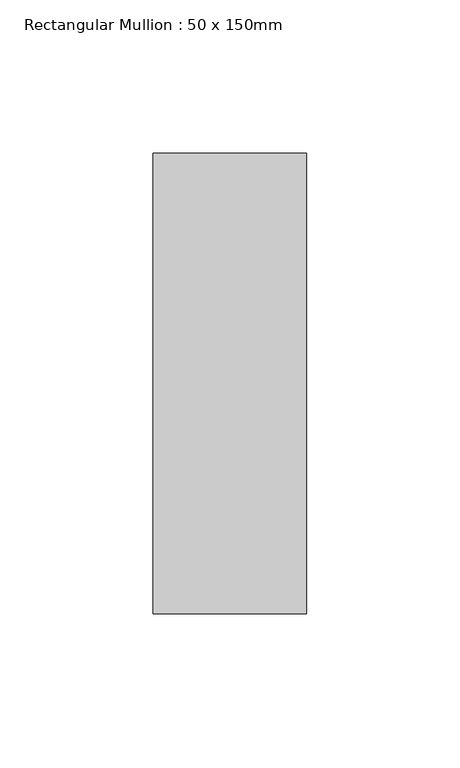
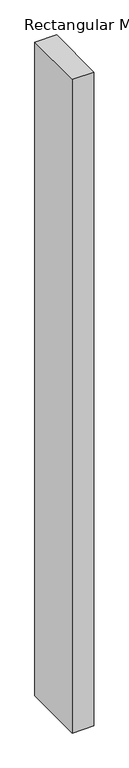
"""IFC4 building model written with IfcOpenShell, lengths in millimetres: member geometry, Rectangular Mullion : 50 x 150mm."""

import ifcopenshell
import ifcopenshell.guid

model = None  # the IFC model being written
_history = None  # IfcOwnerHistory: only IFC2X3 demands one
_inside = {}  # id of a spatial element -> (the spatial element, [elements in it])
_under = {}  # id of a project, library or spatial element -> (it, [spatial elements below it])
_declared = {}  # id of a project -> (the project, [libraries it declares])
_typed = {}  # id of a type object -> (the type object, [elements of that type])
_made_of = {}  # id of a material, layer set ... -> (it, [elements and type objects made of it])


def new_model(schema):
    """Start an empty IFC model of exactly this schema.

    Asked for "IFC4X3", IfcOpenShell would pick the latest addendum, in which some entities
    have other attributes; the version numbers below select the first issue.
    IFC2X3 requires an IfcOwnerHistory on every rooted entity: one is made here for all.
    """
    global model, _history
    if schema == "IFC4X3":
        model = ifcopenshell.file(schema_version=(4, 3, 0, 0))
    else:
        model = ifcopenshell.file(schema=schema)
    _inside.clear()
    _under.clear()
    _declared.clear()
    _typed.clear()
    _made_of.clear()
    _history = None
    if model.schema == "IFC2X3":
        org = make("IfcOrganization", Name="unknown")
        user = make(
            "IfcPersonAndOrganization",
            ThePerson=make("IfcPerson", FamilyName="unknown"),
            TheOrganization=org,
        )
        app = make(
            "IfcApplication",
            ApplicationDeveloper=org,
            Version="unknown",
            ApplicationFullName="unknown",
            ApplicationIdentifier="unknown",
        )
        _history = make(
            "IfcOwnerHistory",
            OwningUser=user,
            OwningApplication=app,
            ChangeAction="ADDED",
            CreationDate=0,
        )
    return model


def make(cls, **values):
    """One entity of the class cls with the attributes given. An attribute that is None is left unset."""
    return model.create_entity(
        cls, **{name: value for name, value in values.items() if value is not None}
    )


def rooted(cls, **values):
    """An entity with a GlobalId (a new one), such as an element, a storey or a relation."""
    return make(cls, GlobalId=ifcopenshell.guid.new(), OwnerHistory=_history, **values)


def si_unit(unit_type, name, prefix=None):
    """IfcSIUnit, for example si_unit("LENGTHUNIT", "METRE", prefix="MILLI")."""
    return make("IfcSIUnit", UnitType=unit_type, Prefix=prefix, Name=name)


def assignment(units):
    """IfcUnitAssignment: the units of a project."""
    return None if units is None else make("IfcUnitAssignment", Units=units)


def point(xyz):
    """IfcCartesianPoint."""
    return None if xyz is None else make("IfcCartesianPoint", Coordinates=xyz)


def direction(xyz):
    """IfcDirection."""
    return None if xyz is None else make("IfcDirection", DirectionRatios=xyz)


def frame(location, z_axis=None, x_axis=None):
    """IfcAxis2Placement3D, a coordinate frame: its origin and axes. An axis left out is left unset."""
    return make(
        "IfcAxis2Placement3D",
        Location=point(location),
        Axis=direction(z_axis),
        RefDirection=direction(x_axis),
    )


def origin():
    """The frame at (0, 0, 0) with its axes left unset."""
    return frame((0.0, 0.0, 0.0))


def place(relative_to, where):
    """IfcLocalPlacement: puts the frame where relative to a parent placement (None: the world)."""
    return make(
        "IfcLocalPlacement", PlacementRelTo=relative_to, RelativePlacement=where
    )


def context(
    kind, dimensions, precision=None, world=None, true_north=None, identifier=None
):
    """IfcGeometricRepresentationContext, for example the 3D "Model" context."""
    return make(
        "IfcGeometricRepresentationContext",
        ContextIdentifier=identifier,
        ContextType=kind,
        CoordinateSpaceDimension=dimensions,
        Precision=precision,
        WorldCoordinateSystem=world,
        TrueNorth=true_north,
    )


def project(units=None, contexts=None):
    """IfcProject with its units and contexts."""
    return rooted(
        "IfcProject",
        Name="project",
        RepresentationContexts=contexts,
        UnitsInContext=assignment(units),
    )


def spatial(cls, under=None, at=None, **own):
    """A site, building, storey or space (cls), placed at a placement, below another one or the project."""
    s = rooted(cls, ObjectPlacement=at, **own)
    if under is not None:
        _under.setdefault(under.id(), (under, []))[1].append(s)
    return s


def polyline(points):
    """IfcPolyline through the points."""
    return make("IfcPolyline", Points=[point(p) for p in points])


def outline(outer, holes=None, kind="AREA"):
    """IfcArbitraryClosedProfileDef: a profile drawn as a closed curve; with holes, ...WithVoids."""
    if holes is None:
        return make("IfcArbitraryClosedProfileDef", ProfileType=kind, OuterCurve=outer)
    return make(
        "IfcArbitraryProfileDefWithVoids",
        ProfileType=kind,
        OuterCurve=outer,
        InnerCurves=holes,
    )


def extrude(swept, where, along, depth):
    """IfcExtrudedAreaSolid: the profile swept, set in the frame where, extruded along a direction by depth."""
    return make(
        "IfcExtrudedAreaSolid",
        SweptArea=swept,
        Position=where,
        ExtrudedDirection=direction(along),
        Depth=depth,
    )


def shape(context_of_items, identifier, shape_type, items):
    """IfcShapeRepresentation: the items that make up one representation, for example the "Body"."""
    return make(
        "IfcShapeRepresentation",
        ContextOfItems=context_of_items,
        RepresentationIdentifier=identifier,
        RepresentationType=shape_type,
        Items=items,
    )


def source(mapping_origin, context_of_items, identifier, shape_type, items):
    """IfcRepresentationMap: a shape defined once, which mapped items show again and again."""
    return make(
        "IfcRepresentationMap",
        MappingOrigin=mapping_origin,
        MappedRepresentation=shape(context_of_items, identifier, shape_type, items),
    )


def transform(
    local_origin,
    x_axis=None,
    y_axis=None,
    z_axis=None,
    scale=None,
    scale2=None,
    scale3=None,
    uniform=True,
):
    """IfcCartesianTransformationOperator3D, or its non-uniform kind. x_axis, y_axis, z_axis: its Axis1, 2, 3."""
    if uniform:
        return make(
            "IfcCartesianTransformationOperator3D",
            Axis1=direction(x_axis),
            Axis2=direction(y_axis),
            LocalOrigin=point(local_origin),
            Scale=scale,
            Axis3=direction(z_axis),
        )
    return make(
        "IfcCartesianTransformationOperator3DnonUniform",
        Axis1=direction(x_axis),
        Axis2=direction(y_axis),
        LocalOrigin=point(local_origin),
        Scale=scale,
        Axis3=direction(z_axis),
        Scale2=scale2,
        Scale3=scale3,
    )


def mapped(mapping_source, mapping_target):
    """IfcMappedItem: shows the shape of a source again, moved by a transform."""
    return make(
        "IfcMappedItem", MappingSource=mapping_source, MappingTarget=mapping_target
    )


def made_of(thing, what):
    """Note that an element or type object is made of a material, layer set ...; save() writes the relation."""
    if what is not None:
        _made_of.setdefault(what.id(), (what, []))[1].append(thing)
    return thing


def element(
    cls,
    number,
    at=None,
    inside=None,
    cuts=None,
    type_object=None,
    material=None,
    context=None,
    identifier="Body",
    shape_type=None,
    held_by="IfcProductDefinitionShape",
    body=None,
    shapes=None,
    **own,
):
    """One element of the class cls, such as IfcWall. Its Tag is "e" and its number.

    at: its placement. inside: the storey or other place that contains it. cuts: it is an
    opening in that element (IfcRelVoidsElement). A single representation is given by context,
    identifier, shape_type and body (its items); several are given by shapes. held_by: the class
    of the entity that holds the representations. save() writes the other relations.
    """
    e = rooted(cls, Tag="e%d" % number, ObjectPlacement=at, **own)
    if body is not None:
        shapes = [shape(context, identifier, shape_type, body)]
    if shapes is not None:
        e.Representation = make(held_by, Representations=shapes)
    if inside is not None:
        _inside.setdefault(inside.id(), (inside, []))[1].append(e)
    if cuts is not None:
        rooted(
            "IfcRelVoidsElement", RelatingBuildingElement=cuts, RelatedOpeningElement=e
        )
    if type_object is not None:
        _typed.setdefault(type_object.id(), (type_object, []))[1].append(e)
    return made_of(e, material)


def aggregate(whole, parts):
    """IfcRelAggregates: a whole, such as a stair, and the parts it consists of."""
    return rooted("IfcRelAggregates", RelatingObject=whole, RelatedObjects=parts)


def save(model, path):
    """Write the relations noted so far, then the file.

    IfcRelAggregates (storeys below a building ...), IfcRelContainedInSpatialStructure (elements
    in a storey), IfcRelDefinesByType, IfcRelAssociatesMaterial and IfcRelDeclares: one each for
    every whole, place, type object, material and project.
    """
    for whole, parts in _under.values():
        aggregate(whole, parts)
    for where, things in _inside.values():
        rooted(
            "IfcRelContainedInSpatialStructure",
            RelatedElements=things,
            RelatingStructure=where,
        )
    for kind, things in _typed.values():
        rooted("IfcRelDefinesByType", RelatedObjects=things, RelatingType=kind)
    for what, things in _made_of.values():
        rooted("IfcRelAssociatesMaterial", RelatedObjects=things, RelatingMaterial=what)
    for by, libraries in _declared.values():
        rooted("IfcRelDeclares", RelatingContext=by, RelatedDefinitions=libraries)
    model.write(path)


def rectangular_mullion_50_x_150mm_319da20d(model_context):
    return source(origin(), model_context, "Body", "SweptSolid", [
        extrude(outline(polyline([(25.0, 75.0), (25.0, -75.0), (-25.0, -75.0), (-25.0, 75.0), (25.0, 75.0)])), frame((0.0, 0.0, -1600.0), z_axis=(0.0, 0.0, 1.0), x_axis=(1.0, 0.0, 0.0)), (0.0, 0.0, 1.0), 1600.0),
    ])


if __name__ == "__main__":
    model = new_model("IFC4")
    model_context = context("Model", 3, world=origin())
    ifc_project = project(units=[si_unit("LENGTHUNIT", "METRE", prefix="MILLI")], contexts=[model_context])
    site = spatial("IfcSite", under=ifc_project)
    building = spatial("IfcBuilding", under=site)
    placement = place(None, origin())
    rectangular_mullion_50_x_150mm_shape = rectangular_mullion_50_x_150mm_319da20d(model_context)
    element("IfcMember", 1, ObjectType="Rectangular Mullion : 50 x 150mm", at=placement, inside=building, context=model_context, shape_type="MappedRepresentation", body=[
        mapped(rectangular_mullion_50_x_150mm_shape, transform((0.0, 0.0, 0.0), x_axis=(1.0, 0.0, 0.0), y_axis=(0.0, 1.0, 0.0), z_axis=(0.0, 0.0, 1.0))),
    ])
    save(model, "model.ifc")

# Revit data of these elements
# Type "Rectangular Mullion : 50 x 150mm"
#   built-in parameter 1007304 = 0.492126 (stored number, unit not read)
#   built-in parameter 1007301 = 0.082021 (stored number, unit not read)
#   built-in parameter 1007300 = 0.082021 (stored number, unit not read)
# Element 1 (IfcMember, "Rectangular Mullion : 50 x 150mm")
#   Materials on its faces: "Metal - Aluminium"
# Materials
#   "Metal - Aluminium": class "Metal", colour RGB 247 247 247, transparency 0
